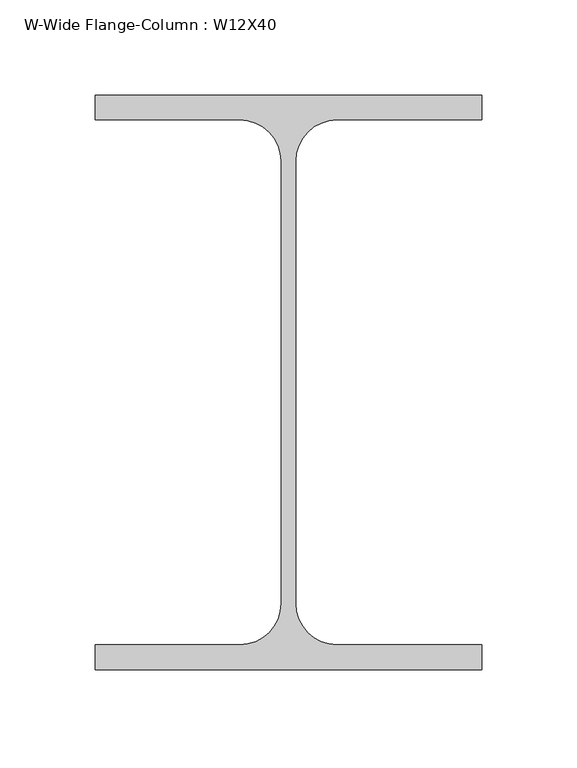
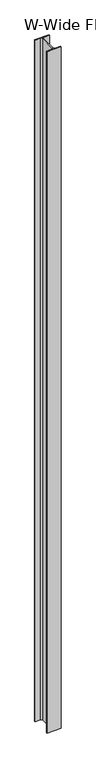
"""IFC4 building model written with IfcOpenShell, lengths in millimetres: column geometry, W-Wide Flange-Column : W12X40."""

from ifc_helpers import new_model, si_unit, point, frame, frame_2d, origin, place, context, project, spatial, polyline, circle_curve, trimmed, segment, composite_curve, outline, extrude, source, transform, mapped, element, save


def w_wide_flange_column_w12x40_c9915c21(model_context):
    return source(origin(), model_context, "Body", "SweptSolid", [
        extrude(outline(composite_curve([segment(polyline([(101.727, 151.13), (101.727, 138.049), (25.5905, 138.049)]), True, "CONTINUOUS"), segment(trimmed(circle_curve(frame_2d((25.5905, 116.205)), 21.844), [point((25.5905, 138.049))], [point((3.7465, 116.205))], True, "CARTESIAN"), True, "CONTINUOUS"), segment(polyline([(3.7465, 116.205), (3.7465, -116.205)]), True, "CONTINUOUS"), segment(trimmed(circle_curve(frame_2d((25.5905, -116.205)), 21.844), [point((3.7465, -116.205))], [point((25.5905, -138.049))], True, "CARTESIAN"), True, "CONTINUOUS"), segment(polyline([(25.5905, -138.049), (101.727, -138.049), (101.727, -151.13), (-101.727, -151.13), (-101.727, -138.049), (-25.5905, -138.049)]), True, "CONTINUOUS"), segment(trimmed(circle_curve(frame_2d((-25.5905, -116.205)), 21.844), [point((-25.5905, -138.049))], [point((-3.7465, -116.205))], True, "CARTESIAN"), True, "CONTINUOUS"), segment(polyline([(-3.7465, -116.205), (-3.7465, 116.205)]), True, "CONTINUOUS"), segment(trimmed(circle_curve(frame_2d((-25.5905, 116.205)), 21.844), [point((-3.7465, 116.205))], [point((-25.5905, 138.049))], True, "CARTESIAN"), True, "CONTINUOUS"), segment(polyline([(-25.5905, 138.049), (-101.727, 138.049), (-101.727, 151.13), (101.727, 151.13)]), True, "CONTINUOUS")], self_intersect=False)), frame((0.0, 0.0, 11550.65), z_axis=(0.0, 0.0, 1.0), x_axis=(1.0, 0.0, 0.0)), (0.0, 0.0, 1.0), 10344.15),
    ])


if __name__ == "__main__":
    model = new_model("IFC4")
    model_context = context("Model", 3, world=origin())
    ifc_project = project(units=[si_unit("LENGTHUNIT", "METRE", prefix="MILLI")], contexts=[model_context])
    site = spatial("IfcSite", under=ifc_project)
    building = spatial("IfcBuilding", under=site)
    placement = place(None, origin())
    w_wide_flange_column_w12x40_shape = w_wide_flange_column_w12x40_c9915c21(model_context)
    element("IfcColumn", 1, ObjectType="W-Wide Flange-Column : W12X40", at=placement, inside=building, context=model_context, shape_type="MappedRepresentation", body=[
        mapped(w_wide_flange_column_w12x40_shape, transform((0.0, 0.0, 0.0), x_axis=(1.0, 0.0, 0.0), y_axis=(0.0, 1.0, 0.0), z_axis=(0.0, 0.0, 1.0))),
    ])
    save(model, "model.ifc")

# Revit data of these elements
# Type "W-Wide Flange-Column : W12X40"
#   Assembly Code = "B10"
#   W = 40
#   bf = 0' - 8.01"
#   d = 0' - 11.9"
#   k = 0' - 1 3/8"
#   kr = 0' - 0.86"
#   tf = 0' - 0.515"
#   tw = 0' - 0.295"
#   A = 0.08125 SF
#   Structural Material [instance default] = Steel ASTM A992
# Element 1 (IfcColumn, "W-Wide Flange-Column : W12X40")
#   Materials on its faces: "Steel ASTM A992"
# Materials
#   "Steel ASTM A992": class "Metal", colour RGB 199 199 199, transparency 0, Description = "Structural steel 50ksi", Cost = 0
